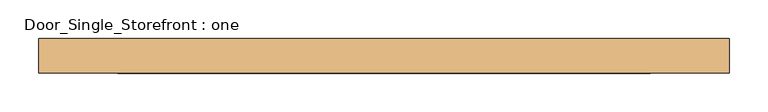
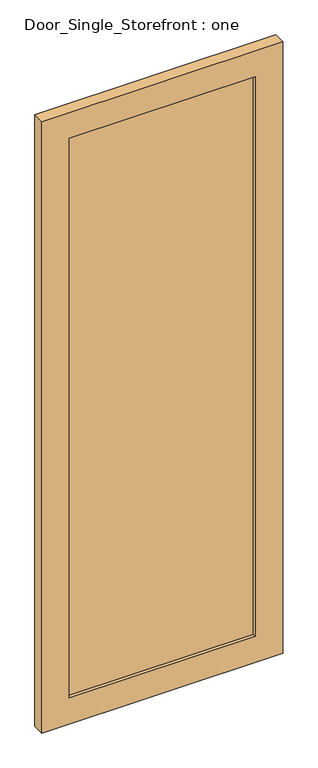
"""IFC4 building model written with IfcOpenShell, lengths in millimetres: door geometry, Door_Single_Storefront : one."""

from ifc_helpers import new_model, si_unit, frame, origin, place, context, project, spatial, polyline, outline, extrude, source, transform, mapped, element, save


def door_single_storefront_one_d0e3d7c8(model_context):
    return source(origin(), model_context, "Body", "SweptSolid", [
        extrude(outline(polyline([(2387.6, -444.5), (0.0, -444.5), (0.0, 444.5), (2387.6, 444.5), (2387.6, -444.5)]), holes=[polyline([(101.6, 342.9), (101.6, -342.9), (2286.0, -342.9), (2286.0, 342.9), (101.6, 342.9)])]), frame((0.0, -19.05, 0.0), z_axis=(0.0, 1.0, 0.0), x_axis=(0.0, 0.0, 1.0)), (0.0, 0.0, 1.0), 44.45),
        extrude(outline(polyline([(342.9, -6.35), (-342.9, -6.35), (-342.9, 12.7), (342.9, 12.7), (342.9, -6.35)])), frame((0.0, 0.0, 101.6), z_axis=(0.0, 0.0, 1.0), x_axis=(1.0, 0.0, 0.0)), (0.0, 0.0, 1.0), 2184.4),
    ])


if __name__ == "__main__":
    model = new_model("IFC4")
    model_context = context("Model", 3, world=origin())
    ifc_project = project(units=[si_unit("LENGTHUNIT", "METRE", prefix="MILLI")], contexts=[model_context])
    site = spatial("IfcSite", under=ifc_project)
    building = spatial("IfcBuilding", under=site)
    placement = place(None, origin())
    door_single_storefront_one_shape = door_single_storefront_one_d0e3d7c8(model_context)
    element("IfcDoor", 1, ObjectType="Door_Single_Storefront : one", at=placement, inside=building, context=model_context, shape_type="MappedRepresentation", body=[
        mapped(door_single_storefront_one_shape, transform((0.0, 0.0, 0.0), x_axis=(1.0, 0.0, 0.0), y_axis=(0.0, 1.0, 0.0), z_axis=(0.0, 0.0, 1.0))),
    ])
    save(model, "model.ifc")

# Revit data of these elements
# Type "Door_Single_Storefront : one"
#   Type Mark = "27"
#   Analytic Construction = "<None>"
#   Stile_Width = 0' - 4"
#   Door_Thickness = 0' - 1 3/4"
#   Door_Offset = 0' - 1"
#   Glass_Material = Glass
#   Frame_Material = Aluminum
#   Function = (empty or 0)
# Element 1 (IfcDoor, "Door_Single_Storefront : one")
#   Materials on its faces: "Aluminum", "Glass"
# Materials
#   "Glass": class "Glass", colour RGB 142 168 196, transparency 0.75, Description = "Soda Lime Glass", Cost = 0
#   "Aluminum": class "Metal", colour RGB 226 226 226, transparency 0, Description = "Aluminum 6061", Cost = 0
